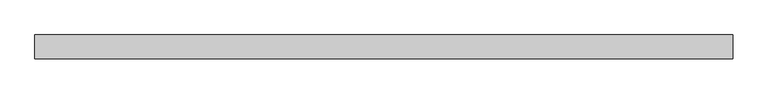
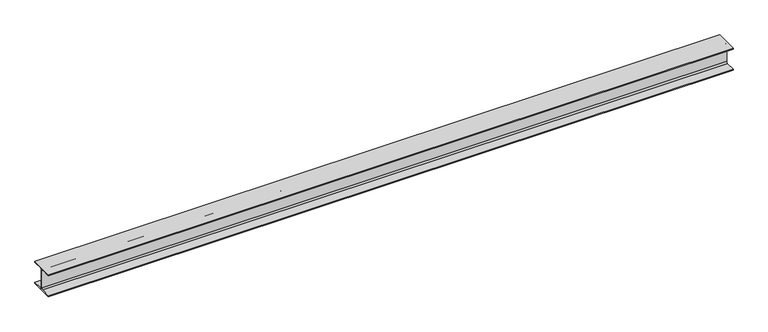
"""IFC4 building model written with IfcOpenShell, lengths in millimetres: beam geometry, 0912_Steel Framing_H-KSD3502 : H_SB_ASB_H-300x300x10x15."""

from ifc_helpers import new_model, si_unit, point, frame, frame_2d, origin, place, context, project, spatial, polyline, circle_curve, trimmed, segment, composite_curve, outline, extrude, source, transform, mapped, element, save


def beam_61b6e8bf(model_context):
    return source(origin(), model_context, "Body", "SweptSolid", [
        extrude(outline(composite_curve([segment(polyline([(150.0, -135.0), (150.0, -150.0), (-150.0, -150.0), (-150.0, -135.0), (-23.0, -135.0)]), True, "CONTINUOUS"), segment(trimmed(circle_curve(frame_2d((-23.0, -117.0)), 18.0), [point((-23.0, -135.0))], [point((-5.0, -117.0))], True, "CARTESIAN"), True, "CONTINUOUS"), segment(polyline([(-5.0, -117.0), (-5.0, 117.0)]), True, "CONTINUOUS"), segment(trimmed(circle_curve(frame_2d((-23.0, 117.0)), 18.0), [point((-5.0, 117.0))], [point((-23.0, 135.0))], True, "CARTESIAN"), True, "CONTINUOUS"), segment(polyline([(-23.0, 135.0), (-150.0, 135.0), (-150.0, 150.0), (150.0, 150.0), (150.0, 135.0), (23.0, 135.0)]), True, "CONTINUOUS"), segment(trimmed(circle_curve(frame_2d((23.0, 117.0)), 18.0), [point((23.0, 135.0))], [point((5.0, 117.0))], True, "CARTESIAN"), True, "CONTINUOUS"), segment(polyline([(5.0, 117.0), (5.0, -117.0)]), True, "CONTINUOUS"), segment(trimmed(circle_curve(frame_2d((23.0, -117.0)), 18.0), [point((5.0, -117.0))], [point((23.0, -135.0))], True, "CARTESIAN"), True, "CONTINUOUS"), segment(polyline([(23.0, -135.0), (150.0, -135.0)]), True, "CONTINUOUS")], self_intersect=False)), frame((-4522.4440295, 0.0, 0.0), z_axis=(1.0, 0.0, 0.0), x_axis=(0.0, 1.0, 0.0)), (0.0, 0.0, 1.0), 8795.3692077),
    ])


if __name__ == "__main__":
    model = new_model("IFC4")
    model_context = context("Model", 3, world=origin())
    ifc_project = project(units=[si_unit("LENGTHUNIT", "METRE", prefix="MILLI")], contexts=[model_context])
    site = spatial("IfcSite", under=ifc_project)
    building = spatial("IfcBuilding", under=site)
    placement = place(None, origin())
    beam_shape = beam_61b6e8bf(model_context)
    element("IfcBeam", 1, ObjectType="0912_Steel Framing_H-KSD3502 : H_SB_ASB_H-300x300x10x15", at=placement, inside=building, context=model_context, shape_type="MappedRepresentation", body=[
        mapped(beam_shape, transform((0.0, 0.0, 0.0), x_axis=(1.0, 0.0, 0.0), y_axis=(0.0, 1.0, 0.0), z_axis=(0.0, 0.0, 1.0))),
    ])
    save(model, "model.ifc")

# Revit data of these elements
# Type "0912_Steel Framing_H-KSD3502 : H_SB_ASB_H-300x300x10x15"
#   H_WM Code_1 = "S01AA001-00001 | Main Steel Structure Fabrication Work | Shelter/Building | Heavy Steel - Standard (Weight≥90KG/M) | Material: (   )"
#   H_WM Code_2 = "S03AA027-00001 | Main Steel Structure Erection Work | Shelter/Building | Heavy Steel (Weight≥90KG/M) | Material: (   )"
#   H_WM Code_3 = "S01AA010-00001 | Main Steel Structure Fabrication Work | Shelter/Building | Steel Painting/Coating | for Non-Fireproofed Steel Surface, Surface Preparation, Primer, Second & Final Coat | Material: (   )"
#   H_Q'ty Cal Type Tag = "SB-Q2"
#   Width = 30.0 cm
#   Web Thickness = 1.0 cm
#   Web Fillet = 1.8 cm
#   Warping Constant = 1370000.0 cm⁶
#   W = 0
#   Torsional Moment of Inertia = 77.00 cm⁴
#   Section Area = 119.8 cm²
#   Plastic Modulus weak axis = 684.0 cm³
#   Plastic Modulus strong axis = 1500.0 cm³
#   Perimeter = 1.75 m²/m
#   Nominal Weight = 94.00 kgf/m
#   Moment of Inertia weak axis = 6750.00 cm⁴
#   Moment of Inertia strong axis = 20400.00 cm⁴
#   Height = 30.0 cm
#   Flange Thickness = 1.5 cm
#   Elastic Modulus weak axis = 450.0 cm³
#   Elastic Modulus strong axis = 1360.0 cm³
#   Centroid Vertical = 15.0 cm
#   Centroid Horizontal = 15.0 cm
#   Ix = 204000000
#   Length [instance default] = 1.5240 m
#   Zx = 1500000
#   b = 0.3000 m
#   h = 0.3000 m
#   r = 0.0180 m
#   s = 0.0100 m
#   t = 0.0150 m
#   A = 0.01198 m²
#   Structural Material [instance default] = Steel, 45-345
#   Assembly Code = ""
# Element 1 (IfcBeam, "0912_Steel Framing_H-KSD3502 : H_SB_ASB_H-300x300x10x15")
#   Structural Material = none
# Materials
#   "Steel, 45-345": class "Metal", colour RGB 189 187 185, transparency 0, Description = "Steel 345 MPa", Cost = 0
